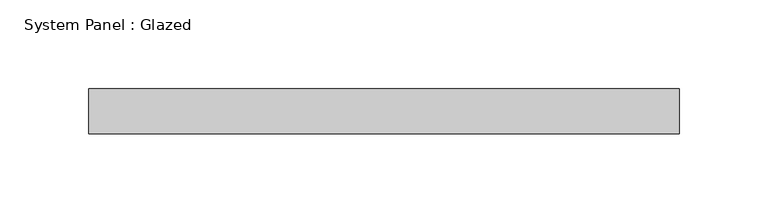
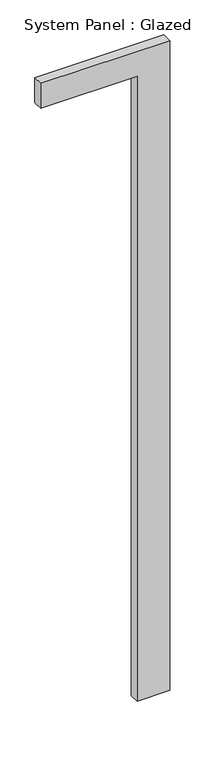
"""IFC4 building model written with IfcOpenShell, lengths in millimetres: plate geometry, System Panel : Glazed."""

from ifc_helpers import new_model, si_unit, frame, origin, place, context, project, spatial, polyline, outline, extrude, source, transform, mapped, element, save


def system_panel_glazed_93cf3d54(model_context):
    return source(origin(), model_context, "Body", "SweptSolid", [
        extrude(outline(polyline([(0.0, 82.55), (0.0, 166.6875), (1774.825, 166.6875), (1774.825, -166.6875), (1706.5625, -166.6875), (1706.5625, 82.55), (0.0, 82.55)])), frame((0.0, -12.7, 0.0), z_axis=(0.0, 1.0, 0.0), x_axis=(0.0, 0.0, 1.0)), (0.0, 0.0, 1.0), 25.4),
    ])


if __name__ == "__main__":
    model = new_model("IFC4")
    model_context = context("Model", 3, world=origin())
    ifc_project = project(units=[si_unit("LENGTHUNIT", "METRE", prefix="MILLI")], contexts=[model_context])
    site = spatial("IfcSite", under=ifc_project)
    building = spatial("IfcBuilding", under=site)
    placement = place(None, origin())
    system_panel_glazed_shape = system_panel_glazed_93cf3d54(model_context)
    element("IfcPlate", 1, ObjectType="System Panel : Glazed", at=placement, inside=building, context=model_context, shape_type="MappedRepresentation", body=[
        mapped(system_panel_glazed_shape, transform((0.0, 0.0, 0.0), x_axis=(1.0, 0.0, 0.0), y_axis=(0.0, 1.0, 0.0), z_axis=(0.0, 0.0, 1.0))),
    ])
    save(model, "model.ifc")

# Revit data of these elements
# Element 1 (IfcPlate, "System Panel : Glazed")
#   Materials on its faces: "EXISTING GLAZING AND STOREFRONT"
# Materials
#   "EXISTING GLAZING AND STOREFRONT": class "Glass", colour RGB 218 227 224, transparency 0.85, Description = "Soda Lime Glass", Cost = 0
